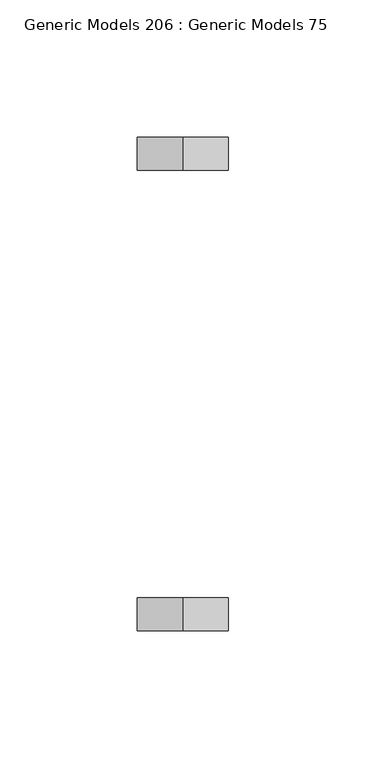
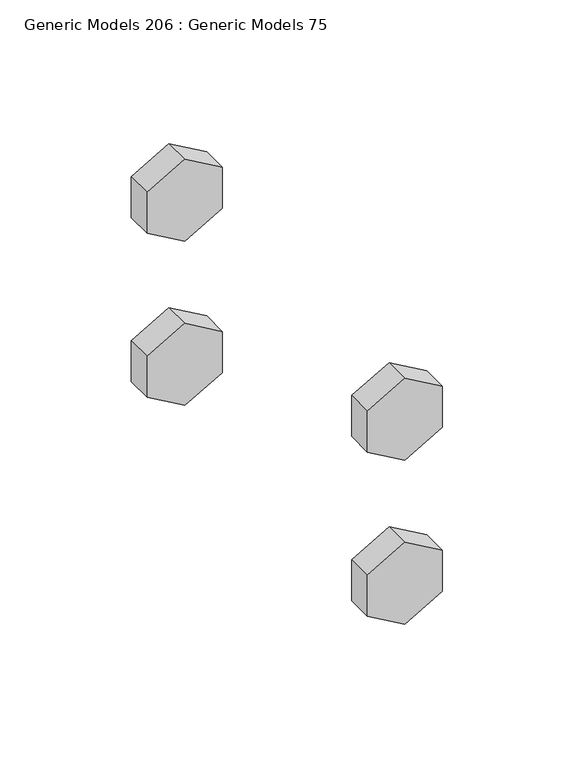
"""IFC4 building model written with IfcOpenShell, lengths in millimetres: proxy geometry, Generic Models 206 : Generic Models 75."""

from ifc_helpers import new_model, si_unit, frame, origin, place, context, project, spatial, polyline, outline, extrude, source, transform, mapped, element, save


def generic_models_206_generic_models_75_f2be38f4(model_context):
    return source(origin(), model_context, "Body", "SweptSolid", [
        extrude(outline(polyline([(271679.9875, 31991.9073871), (271699.0375, 31991.9073871), (271708.5625, 31975.4096032), (271699.0375, 31958.9118192), (271679.9875, 31958.9118192), (271670.4625, 31975.4096032), (271679.9875, 31991.9073871)])), frame((0.0, 36485.2082942, 0.0), z_axis=(0.0, 1.0, 0.0), x_axis=(0.0, 0.0, 1.0)), (0.0, 0.0, 1.0), 11.90625),
        extrude(outline(polyline([(271603.7875, 31991.9073871), (271622.8375, 31991.9073871), (271632.3625, 31975.4096032), (271622.8375, 31958.9118192), (271603.7875, 31958.9118192), (271594.2625, 31975.4096032), (271603.7875, 31991.9073871)])), frame((0.0, 36485.2082942, 0.0), z_axis=(0.0, 1.0, 0.0), x_axis=(0.0, 0.0, 1.0)), (0.0, 0.0, 1.0), 11.90625),
        extrude(outline(polyline([(271679.9875, 31991.9073871), (271699.0375, 31991.9073871), (271708.5625, 31975.4096032), (271699.0375, 31958.9118192), (271679.9875, 31958.9118192), (271670.4625, 31975.4096032), (271679.9875, 31991.9073871)])), frame((0.0, 36317.7270442, 0.0), z_axis=(0.0, 1.0, 0.0), x_axis=(0.0, 0.0, 1.0)), (0.0, 0.0, 1.0), 11.90625),
        extrude(outline(polyline([(271603.7875, 31991.9073871), (271622.8375, 31991.9073871), (271632.3625, 31975.4096032), (271622.8375, 31958.9118192), (271603.7875, 31958.9118192), (271594.2625, 31975.4096032), (271603.7875, 31991.9073871)])), frame((0.0, 36317.7270442, 0.0), z_axis=(0.0, 1.0, 0.0), x_axis=(0.0, 0.0, 1.0)), (0.0, 0.0, 1.0), 11.90625),
    ])


if __name__ == "__main__":
    model = new_model("IFC4")
    model_context = context("Model", 3, world=origin())
    ifc_project = project(units=[si_unit("LENGTHUNIT", "METRE", prefix="MILLI")], contexts=[model_context])
    site = spatial("IfcSite", under=ifc_project)
    building = spatial("IfcBuilding", under=site)
    placement = place(None, origin())
    generic_models_206_generic_models_75_shape = generic_models_206_generic_models_75_f2be38f4(model_context)
    element("IfcBuildingElementProxy", 1, Name="Generic Models 206 : Generic Models 75", ObjectType="Generic Models 206 : Generic Models 75", at=placement, inside=building, context=model_context, shape_type="MappedRepresentation", body=[
        mapped(generic_models_206_generic_models_75_shape, transform((0.0, 0.0, 0.0), x_axis=(1.0, 0.0, 0.0), y_axis=(0.0, 1.0, 0.0), z_axis=(0.0, 0.0, 1.0))),
    ])
    save(model, "model.ifc")
